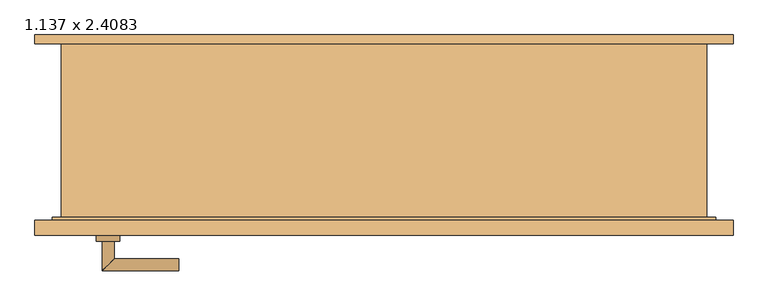
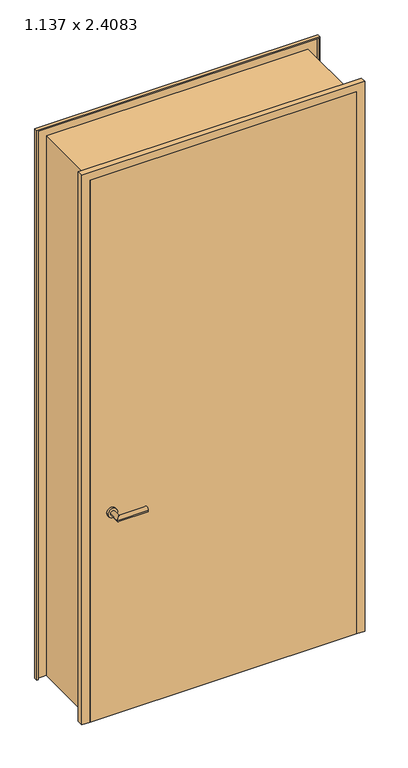
"""IFC4 building model written with IfcOpenShell, lengths in millimetres: door geometry, Drehflügel 1-flg - Stahlzarge : 1.137 x 2.4083."""

from ifc_helpers import new_model, si_unit, point, frame, frame_2d, origin, place, context, project, spatial, polyline, circle_curve, ellipse_curve, trimmed, segment, composite_curve, outline, extrude, faceted_brep, source, transform, mapped, element, save
from ifc_brep_helpers import plane_surface, cylinder_surface, advanced_brep


def door_1_137_x_2_4083_9fef643e(model_context):
    return source(origin(), model_context, "Body", "SolidModel", [
        advanced_brep(
        [(-478.5, -139.4346141, 915.0), (-458.5, -139.4346141, 915.0), (-458.5, -89.4346141, 915.0), (-478.5, -69.4346141, 915.0), (-348.5, -69.4346141, 915.0), (-348.5, -89.4346141, 915.0)],
        [
            (0, 1, circle_curve(frame((-468.5, -139.4346141, 915.0), z_axis=(0.0, -1.0, 0.0), x_axis=(1.0, 0.0, 0.0)), 10.0)),
            (1, 0, circle_curve(frame((-468.5, -139.4346141, 915.0), z_axis=(0.0, -1.0, 0.0), x_axis=(1.0, 0.0, 0.0)), 10.0)),
            (1, 2),
            (2, 3, ellipse_curve(frame((-468.5, -79.4346141, 915.0), z_axis=(-0.7071067811865385, -0.7071067811865565, 0.0), x_axis=(0.7071067811865563, -0.7071067811865386, 0.0)), 14.1421356, 10.0)),
            (3, 0),
            (3, 2, ellipse_curve(frame((-468.5, -79.4346141, 915.0), z_axis=(-0.7071067811865385, -0.7071067811865565, 0.0), x_axis=(0.7071067811865563, -0.7071067811865386, 0.0)), 14.1421356, 10.0)),
            (4, 5, circle_curve(frame((-348.5, -79.4346141, 915.0), z_axis=(1.0, 0.0, 0.0), x_axis=(0.0, -1.0, 0.0)), 10.0)),
            (5, 4, circle_curve(frame((-348.5, -79.4346141, 915.0), z_axis=(1.0, 0.0, 0.0), x_axis=(0.0, -1.0, 0.0)), 10.0)),
            (2, 5),
            (4, 3),
        ],
        [
            plane_surface(frame((-468.5, -139.4346141, -372.7526403), z_axis=(0.0, -1.0, 0.0), x_axis=(0.0, 0.0, 1.0))),
            cylinder_surface(frame((-468.5, -139.4346141, 915.0), z_axis=(0.0, -1.0, 0.0), x_axis=(1.0, 0.0, 0.0)), 10.0),
            plane_surface(frame((-348.5, -79.4346141, -372.7526403), z_axis=(1.0, 0.0, 0.0), x_axis=(0.0, 0.0, 1.0))),
            cylinder_surface(frame((-468.5, -79.4346141, 915.0), z_axis=(-1.0, 0.0, 0.0), x_axis=(0.0, -1.0, 0.0)), 10.0),
        ],
        [
            (0, [[1, 2]]),
            (1, [[3, 4, 5, -2]]),
            (1, [[-5, 6, -3, -1]]),
            (2, [[7, 8]]),
            (3, [[9, -7, 10, -4]]),
            (3, [[-10, -8, -9, -6]]),
        ],
    ),
        advanced_brep(
        [(-458.5, -199.4346141, 915.0), (-478.5, -199.4346141, 915.0), (-478.5, -249.4346141, 915.0), (-458.5, -229.4346141, 915.0), (-348.5, -229.4346141, 915.0), (-348.5, -249.4346141, 915.0)],
        [
            (0, 1, circle_curve(frame((-468.5, -199.4346141, 915.0), z_axis=(0.0, 1.0, 0.0), x_axis=(-1.0, 0.0, 0.0)), 10.0)),
            (1, 0, circle_curve(frame((-468.5, -199.4346141, 915.0), z_axis=(0.0, 1.0, 0.0), x_axis=(-1.0, 0.0, 0.0)), 10.0)),
            (1, 2),
            (2, 3, ellipse_curve(frame((-468.5, -239.4346141, 915.0), z_axis=(-0.7071067811865475, 0.7071067811865475, 0.0), x_axis=(0.7071067811865474, 0.7071067811865476, 0.0)), 14.1421356, 10.0)),
            (3, 0),
            (3, 2, ellipse_curve(frame((-468.5, -239.4346141, 915.0), z_axis=(-0.7071067811865475, 0.7071067811865475, 0.0), x_axis=(0.7071067811865474, 0.7071067811865476, 0.0)), 14.1421356, 10.0)),
            (4, 5, circle_curve(frame((-348.5, -239.4346141, 915.0), z_axis=(1.0, 0.0, 0.0), x_axis=(0.0, -1.0, 0.0)), 10.0)),
            (5, 4, circle_curve(frame((-348.5, -239.4346141, 915.0), z_axis=(1.0, 0.0, 0.0), x_axis=(0.0, -1.0, 0.0)), 10.0)),
            (2, 5),
            (4, 3),
        ],
        [
            plane_surface(frame((-468.5, -199.4346141, -372.7526403), z_axis=(0.0, 1.0, 0.0), x_axis=(0.0, 0.0, 1.0))),
            cylinder_surface(frame((-468.5, -199.4346141, 915.0), z_axis=(0.0, 1.0, 0.0), x_axis=(-1.0, 0.0, 0.0)), 10.0),
            plane_surface(frame((-348.5, -239.4346141, -372.7526403), z_axis=(1.0, 0.0, 0.0), x_axis=(0.0, 0.0, 1.0))),
            cylinder_surface(frame((-468.5, -239.4346141, 915.0), z_axis=(-1.0, 0.0, 0.0), x_axis=(0.0, -1.0, 0.0)), 10.0),
        ],
        [
            (0, [[1, 2]]),
            (1, [[3, 4, 5, -2]]),
            (1, [[-5, 6, -3, -1]]),
            (2, [[7, 8]]),
            (3, [[9, -7, 10, -4]]),
            (3, [[-10, -8, -9, -6]]),
        ],
    ),
        extrude(outline(composite_curve([segment(trimmed(circle_curve(frame_2d((915.0, -468.5)), 20.0), [point((915.0, -488.5))], [point((915.0, -448.5))], False, "CARTESIAN"), True, "CONTINUOUS"), segment(trimmed(circle_curve(frame_2d((915.0, -468.5)), 20.0), [point((915.0, -448.5))], [point((915.0, -488.5))], False, "CARTESIAN"), True, "CONTINUOUS")], self_intersect=False)), frame((0.0, -139.4346141, 0.0), z_axis=(0.0, 1.0, 0.0), x_axis=(0.0, 0.0, 1.0)), (0.0, 0.0, 1.0), 10.0),
        extrude(outline(composite_curve([segment(trimmed(circle_curve(frame_2d((915.0, -468.5)), 20.0), [point((915.0, -488.5))], [point((915.0, -448.5))], False, "CARTESIAN"), True, "CONTINUOUS"), segment(trimmed(circle_curve(frame_2d((915.0, -468.5)), 20.0), [point((915.0, -448.5))], [point((915.0, -488.5))], False, "CARTESIAN"), True, "CONTINUOUS")], self_intersect=False)), frame((0.0, -199.4346141, 0.0), z_axis=(0.0, 1.0, 0.0), x_axis=(0.0, 0.0, 1.0)), (0.0, 0.0, 1.0), 10.0),
        extrude(outline(polyline([(558.5, -164.4346141), (558.5, -189.4346141), (-558.5, -189.4346141), (-558.5, -164.4346141), (558.5, -164.4346141)])), frame((0.0, 0.0, 15.0), z_axis=(0.0, 0.0, 1.0), x_axis=(1.0, 0.0, 0.0)), (0.0, 0.0, 1.0), 2398.3),
        faceted_brep([(592.9603207, 150.5653859, 15.0), (592.9603207, 135.5653859, 15.0), (587.9603207, 135.5653859, 15.0), (587.9603207, 145.5653859, 15.0), (548.5, 145.5653859, 15.0), (548.5, -159.4346141, 15.0), (563.5, -159.4346141, 15.0), (563.5, -184.4346141, 15.0), (587.9603207, -184.4346141, 15.0), (587.9603207, -164.4346141, 15.0), (592.9603207, -164.4346141, 15.0), (592.9603207, -189.4346141, 15.0), (558.5, -189.4346141, 15.0), (558.5, -164.4346141, 15.0), (543.5, -164.4346141, 15.0), (543.5, 150.5653859, 15.0), (543.5, 150.5653859, 2398.3), (-543.5, 150.5653859, 2398.3), (-543.5, 150.5653859, 15.0), (-592.9603207, 150.5653859, 15.0), (-592.9603207, 150.5653859, 2447.7603207), (592.9603207, 150.5653859, 2447.7603207), (543.5, -164.4346141, 2398.3), (558.5, -164.4346141, 2413.3), (-558.5, -164.4346141, 2413.3), (-558.5, -164.4346141, 15.0), (-543.5, -164.4346141, 15.0), (-543.5, -164.4346141, 2398.3), (558.5, -189.4346141, 2413.3), (592.9603207, -189.4346141, 2447.7603207), (-592.9603207, -189.4346141, 2447.7603207), (-592.9603207, -189.4346141, 15.0), (-558.5, -189.4346141, 15.0), (-558.5, -189.4346141, 2413.3), (592.9603207, -164.4346141, 2447.7603207), (587.9603207, -164.4346141, 2442.7603207), (-587.9603207, -164.4346141, 2442.7603207), (-587.9603207, -164.4346141, 15.0), (-592.9603207, -164.4346141, 15.0), (-592.9603207, -164.4346141, 2447.7603207), (587.9603207, -184.4346141, 2442.7603207), (563.5, -184.4346141, 2418.3), (-563.5, -184.4346141, 2418.3), (-563.5, -184.4346141, 15.0), (-587.9603207, -184.4346141, 15.0), (-587.9603207, -184.4346141, 2442.7603207), (563.5, -159.4346141, 2418.3), (548.5, -159.4346141, 2403.3), (-548.5, -159.4346141, 2403.3), (-548.5, -159.4346141, 15.0), (-563.5, -159.4346141, 15.0), (-563.5, -159.4346141, 2418.3), (548.5, 145.5653859, 2403.3), (587.9603207, 145.5653859, 2442.7603207), (-587.9603207, 145.5653859, 2442.7603207), (-587.9603207, 145.5653859, 15.0), (-548.5, 145.5653859, 15.0), (-548.5, 145.5653859, 2403.3), (587.9603207, 135.5653859, 2442.7603207), (592.9603207, 135.5653859, 2447.7603207), (-592.9603207, 135.5653859, 2447.7603207), (-592.9603207, 135.5653859, 15.0), (-587.9603207, 135.5653859, 15.0), (-587.9603207, 135.5653859, 2442.7603207)], [[[0, 1, 2, 3, 4, 5, 6, 7, 8, 9, 10, 11, 12, 13, 14, 15]], [[15, 16, 17, 18, 19, 20, 21, 0]], [[14, 22, 16, 15]], [[13, 23, 24, 25, 26, 27, 22, 14]], [[12, 28, 23, 13]], [[11, 29, 30, 31, 32, 33, 28, 12]], [[10, 34, 29, 11]], [[9, 35, 36, 37, 38, 39, 34, 10]], [[8, 40, 35, 9]], [[7, 41, 42, 43, 44, 45, 40, 8]], [[6, 46, 41, 7]], [[5, 47, 48, 49, 50, 51, 46, 6]], [[4, 52, 47, 5]], [[3, 53, 54, 55, 56, 57, 52, 4]], [[2, 58, 53, 3]], [[1, 59, 60, 61, 62, 63, 58, 2]], [[0, 21, 59, 1]], [[20, 19, 61, 60]], [[19, 18, 26, 25, 32, 31, 38, 37, 44, 43, 50, 49, 56, 55, 62, 61]], [[27, 26, 18, 17]], [[33, 32, 25, 24]], [[39, 38, 31, 30]], [[45, 44, 37, 36]], [[51, 50, 43, 42]], [[57, 56, 49, 48]], [[63, 62, 55, 54]], [[22, 27, 17, 16]], [[28, 33, 24, 23]], [[34, 39, 30, 29]], [[40, 45, 36, 35]], [[46, 51, 42, 41]], [[52, 57, 48, 47]], [[58, 63, 54, 53]], [[21, 20, 60, 59]]]),
    ])


if __name__ == "__main__":
    model = new_model("IFC4")
    model_context = context("Model", 3, world=origin())
    ifc_project = project(units=[si_unit("LENGTHUNIT", "METRE", prefix="MILLI")], contexts=[model_context])
    site = spatial("IfcSite", under=ifc_project)
    building = spatial("IfcBuilding", under=site)
    placement = place(None, origin())
    door_1_137_x_2_4083_shape = door_1_137_x_2_4083_9fef643e(model_context)
    element("IfcDoor", 1, ObjectType="Drehflügel 1-flg - Stahlzarge : 1.137 x 2.4083", at=placement, inside=building, context=model_context, shape_type="MappedRepresentation", body=[
        mapped(door_1_137_x_2_4083_shape, transform((0.0, 0.0, 0.0), x_axis=(1.0, 0.0, 0.0), y_axis=(0.0, 1.0, 0.0), z_axis=(0.0, 0.0, 1.0))),
    ])
    save(model, "model.ifc")

# Revit data of these elements
# Type "Drehflügel 1-flg - Stahlzarge : 1.137 x 2.4083"
#   Type Mark = "21"
#   Operation = "SingleSwingRight"
#   Keynote = "16.03"
#   Analytic Construction = "Metall"
#   Thermal Resistance (R) = 0.270117 (m²·K)/W
#   Heat Transfer Coefficient (U) = 3.7021 W/(m²·K)
#   Rough Width = 1.137 m
#   Rough Height [instance default] = 2.5083 m
#   Höhe Türgriff [instance default] = 0.900 m
#   Height = 2.4083 m
#   Fußbodenaufbau [instance default] = 0.100 m
#   Width = 1.137 m
#   Sichtbarkeit Sturzlinien [instance default] = yes
#   Türgriff auswählen [instance default] = element 221079
#   Türgriff [instance default] = none
#   Türflügel [instance default] = none
#   Rahmen/Pfosten [instance default] = Metall - Lackiert - Grau
#   Visual Light Transmittance = 0
#   Solar Heat Gain Coefficient = 0
#   Function = (empty or 0)
#   Wall Closure = (empty or 0)
# Element 1 (IfcDoor, "Drehflügel 1-flg - Stahlzarge : 1.137 x 2.4083")
#   Rough Height = 2.4233 m
#   Fußbodenaufbau = 0.015 m
#   Materials on its faces: "Metall - Lackiert - Grau", "Metall - Chrom", "Holz - Birke"
# Materials
#   "Metall - Lackiert - Grau": class "Farbe 1", colour RGB 98 98 98, transparency 0, Cost = 0
#   "Metall - Chrom": class "Metall", colour RGB 247 247 247, transparency 0, Cost = 0
#   "Holz - Birke": class "Holz", colour RGB 213 164 103, transparency 0, Cost = 0
